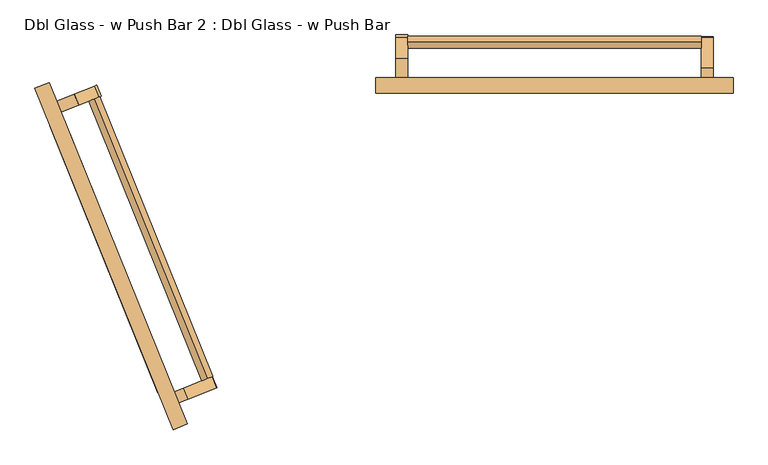
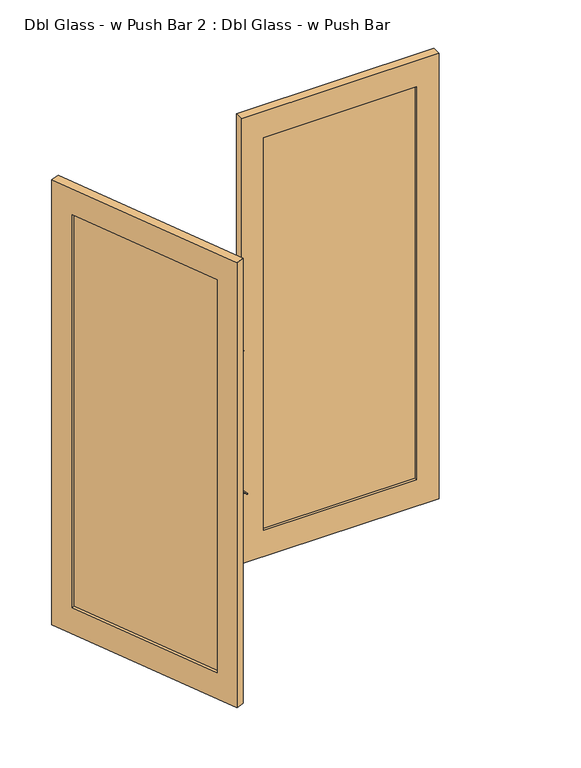
"""IFC4 building model written with IfcOpenShell, lengths in millimetres: door geometry, Dbl Glass - w Push Bar 2 : Dbl Glass - w Push Bar."""

from ifc_helpers import new_model, si_unit, point, frame, frame_2d, origin, place, context, project, spatial, polyline, circle_curve, trimmed, segment, composite_curve, outline, extrude, source, transform, mapped, element, save


def dbl_glass_w_push_bar_2_dbl_glass_w_push_bar_dfafdb44(model_context):
    return source(origin(), model_context, "Body", "SweptSolid", [
        extrude(outline(composite_curve([segment(trimmed(circle_curve(frame_2d((65.0203019, 954.5721086)), 15.0), [point((65.0203019, 969.5721086))], [point((65.0203019, 939.5721086))], False, "CARTESIAN"), True, "CONTINUOUS"), segment(trimmed(circle_curve(frame_2d((65.0203019, 954.5721086)), 15.0), [point((65.0203019, 939.5721086))], [point((65.0203019, 969.5721086))], False, "CARTESIAN"), True, "CONTINUOUS")], self_intersect=False)), frame((80.0, 0.0, 0.0), z_axis=(1.0, 0.0, 0.0), x_axis=(0.0, 1.0, 0.0)), (0.0, 0.0, 1.0), 731.0),
        extrude(outline(composite_curve([segment(polyline([(-0.1563269, 1000.0), (77.6459332, 922.19774)]), True, "CONTINUOUS"), segment(trimmed(circle_curve(frame_2d((75.7878695, 920.3396763)), 2.6276989), [point((77.6459332, 922.19774))], [point((73.9298058, 918.4816126))], False, "CARTESIAN"), True, "CONTINUOUS"), segment(polyline([(73.9298058, 918.4816126), (57.4114184, 935.0), (-24.035259, 935.0), (-24.035259, 1000.0), (-0.1563269, 1000.0)]), True, "CONTINUOUS")], self_intersect=False)), frame((811.0, 0.0, 0.0), z_axis=(1.0, 0.0, 0.0), x_axis=(0.0, 1.0, 0.0)), (0.0, 0.0, 1.0), 30.0),
        extrude(outline(composite_curve([segment(polyline([(23.375226, 1000.0), (77.6459332, 945.7292928)]), True, "CONTINUOUS"), segment(trimmed(circle_curve(frame_2d((65.0203019, 933.1036615)), 17.8553391), [point((77.6459332, 945.7292928))], [point((52.3946705, 920.4780301))], False, "CARTESIAN"), True, "CONTINUOUS"), segment(polyline([(52.3946705, 920.4780301), (37.8727007, 935.0), (-24.035259, 935.0), (-24.035259, 1000.0), (23.375226, 1000.0)]), True, "CONTINUOUS")], self_intersect=False)), frame((50.0, 0.0, 0.0), z_axis=(1.0, 0.0, 0.0), x_axis=(0.0, 1.0, 0.0)), (0.0, 0.0, 1.0), 30.0),
        extrude(outline(composite_curve([segment(trimmed(circle_curve(frame_2d((0.0, 15.0)), 15.0), [point((0.0, 30.0))], [point((0.0, 0.0))], False, "CARTESIAN"), True, "CONTINUOUS"), segment(trimmed(circle_curve(frame_2d((0.0, 15.0)), 15.0), [point((0.0, 0.0))], [point((0.0, 30.0))], False, "CARTESIAN"), True, "CONTINUOUS")], self_intersect=False)), frame((-419.6508941, -774.4258968, 939.5721086), z_axis=(-0.37460659341591906, 0.9271838545667846, 0.0), x_axis=(-0.9271838545667846, -0.37460659341591906, 0.0)), (0.0, 0.0, 1.0), 752.3041635),
        extrude(outline(composite_curve([segment(polyline([(23.8789322, 0.0), (0.0, 0.0), (0.0, 65.0), (81.4466774, 65.0), (97.9650649, 81.5183874)]), True, "CONTINUOUS"), segment(trimmed(circle_curve(frame_2d((99.8231285, 79.6603237)), 2.6276989), [point((97.9650649, 81.5183874))], [point((101.6811923, 77.80226))], False, "CARTESIAN"), True, "CONTINUOUS"), segment(polyline([(101.6811923, 77.80226), (23.8789322, 0.0)]), True, "CONTINUOUS")], self_intersect=False)), frame((-490.9835746, -835.6022127, 1000.0), z_axis=(-0.37460659341591906, 0.9271838545667846, 0.0), x_axis=(0.9271838545667846, 0.37460659341591906, 0.0)), (0.0, 0.0, 1.0), 30.0),
        extrude(outline(composite_curve([segment(polyline([(47.4104851, 0.0), (0.0, 0.0), (0.0, 65.0), (61.9079597, 65.0), (76.4299296, 79.5219699)]), True, "CONTINUOUS"), segment(trimmed(circle_curve(frame_2d((89.055561, 66.8963385)), 17.8553391), [point((76.4299296, 79.5219699))], [point((101.6811923, 54.2707072))], False, "CARTESIAN"), True, "CONTINUOUS"), segment(polyline([(101.6811923, 54.2707072), (47.4104851, 0.0)]), True, "CONTINUOUS")], self_intersect=False)), frame((-784.0398723, -110.262423, 1000.0), z_axis=(-0.37460659341591906, 0.9271838545667846, 0.0), x_axis=(0.9271838545667846, 0.37460659341591906, 0.0)), (0.0, 0.0, 1.0), 30.0),
        extrude(outline(polyline([(0.0, 0.0), (-2125.0, 0.0), (-2125.0, 919.2412593), (0.0, 919.2412593), (0.0, 0.0)]), holes=[polyline([(-125.0, 100.0000001), (-125.0, 819.2412594), (-2000.0, 819.2412594), (-2000.0, 100.0000001), (-125.0, 100.0000001)])]), frame((-849.7454002, -50.5264, 2125.0), z_axis=(0.9271838545667834, 0.37460659341592206, 0.0), x_axis=(0.0, 0.0, 1.0)), (0.0, 0.0, 1.0), 38.5435966),
        extrude(outline(polyline([(2125.0, 0.0), (0.0, 0.0), (0.0, 891.0), (2125.0, 891.0), (2125.0, 0.0)]), holes=[polyline([(2000.0, 100.0), (2000.0, 791.0), (125.0, 791.0), (125.0, 100.0), (2000.0, 100.0)])]), frame((0.0, -62.5788556, 0.0), z_axis=(0.0, 1.0, 0.0), x_axis=(0.0, 0.0, 1.0)), (0.0, 0.0, 1.0), 38.5435966),
        extrude(outline(polyline([(-520.0631047, -800.9062673), (-531.189311, -805.4015464), (-800.621829, -138.5326632), (-789.4956227, -134.0373841), (-520.0631047, -800.9062673)])), frame((0.0, 0.0, 125.0), z_axis=(0.0, 0.0, 1.0), x_axis=(1.0, 0.0, 0.0)), (0.0, 0.0, 1.0), 1875.0),
        extrude(outline(polyline([(791.0, -38.0), (791.0, -50.0), (100.0, -50.0), (100.0, -38.0), (791.0, -38.0)])), frame((0.0, 0.0, 125.0), z_axis=(0.0, 0.0, 1.0), x_axis=(1.0, 0.0, 0.0)), (0.0, 0.0, 1.0), 1875.0),
    ])


if __name__ == "__main__":
    model = new_model("IFC4")
    model_context = context("Model", 3, world=origin())
    ifc_project = project(units=[si_unit("LENGTHUNIT", "METRE", prefix="MILLI")], contexts=[model_context])
    site = spatial("IfcSite", under=ifc_project)
    building = spatial("IfcBuilding", under=site)
    placement = place(None, origin())
    dbl_glass_w_push_bar_2_dbl_glass_w_push_bar_shape = dbl_glass_w_push_bar_2_dbl_glass_w_push_bar_dfafdb44(model_context)
    element("IfcDoor", 1, ObjectType="Dbl Glass - w Push Bar 2 : Dbl Glass - w Push Bar", at=placement, inside=building, context=model_context, shape_type="MappedRepresentation", body=[
        mapped(dbl_glass_w_push_bar_2_dbl_glass_w_push_bar_shape, transform((0.0, 0.0, 0.0), x_axis=(1.0, 0.0, 0.0), y_axis=(0.0, 1.0, 0.0), z_axis=(0.0, 0.0, 1.0))),
    ])
    save(model, "model.ifc")

# Revit data of these elements
# Type "Dbl Glass - w Push Bar 2 : Dbl Glass - w Push Bar"
#   Type Mark = "68"
#   Description = "Curtain Wall Door"
#   Construction Type Id = "GSP4R"
#   Analytic Construction = "1/8 in Pilkington single glazing"
#   Visual Light Transmittance = 0.9
#   TopRail = 125 mm
#   Thermal Resistance (R) = 0.271106 (m²·K)/W
#   Solar Heat Gain Coefficient = 0.78
#   Offset = 50 mm
#   MuntinRail = 100 mm
#   LockRail = 100 mm
#   Heat Transfer Coefficient (U) = 3.6886 W/(m²·K)
#   Handle Z Distance = 1000 mm
#   Handle X Offset = 65 mm
#   Glass Thickness = 12 mm
#   BottomRail = 125 mm
#   Define Thermal Properties by = 1
#   Material Ironmongery = Metal - Aluminum
#   Material Door = Metal - Aluminum
#   Material Glass = Glass
#   Function = (empty or 0)
# Element 1 (IfcDoor, "Dbl Glass - w Push Bar 2 : Dbl Glass - w Push Bar")
#   Materials on its faces: "Metal - Aluminum", "Glass"
# Materials
#   "Metal - Aluminum": class "Metal", colour RGB 247 247 247, transparency 0
#   "Glass": class "Glass", colour RGB 0 128 192, transparency 0.9, Description = "Soda Lime Glass", Cost = 0
